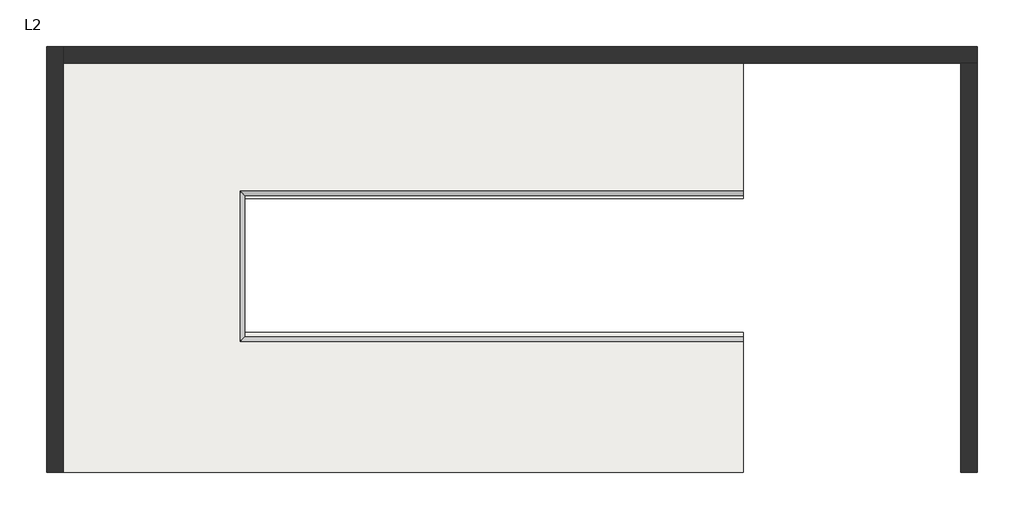
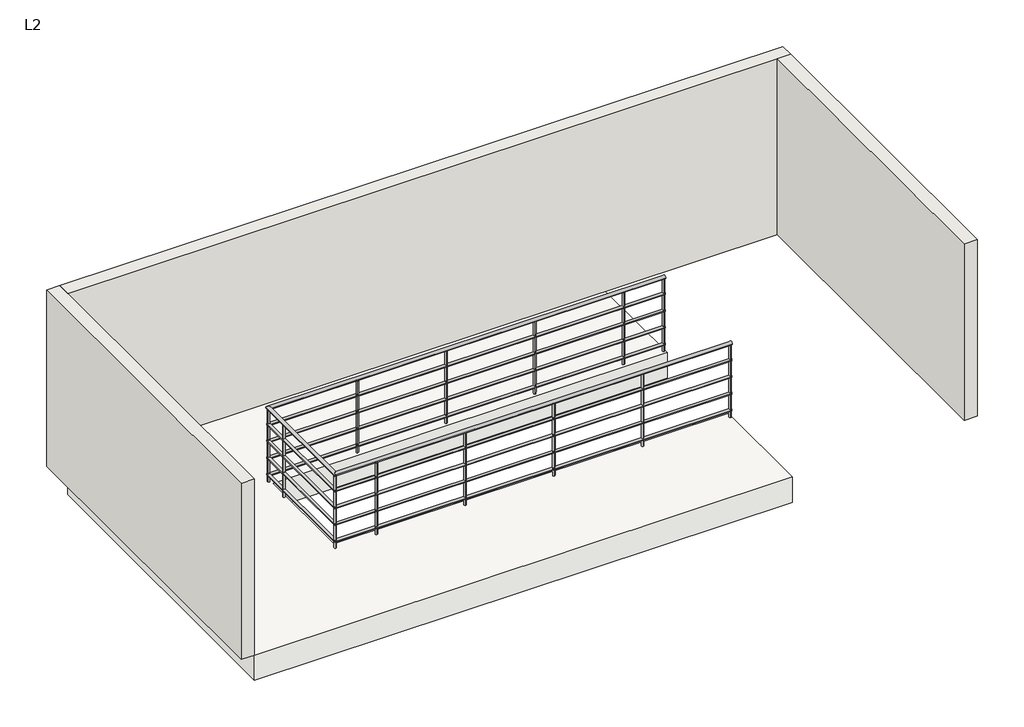
# One storey: 3 walls, 1 railing, 1 slab.
"""IFC4 building model written with IfcOpenShell, lengths in millimetres."""

from ifc_helpers import new_model, si_unit, point, frame, frame_2d, origin, place, context, project, spatial, polyline, circle_curve, ellipse_curve, trimmed, segment, composite_curve, outline, extrude, faceted_brep, element, save
from ifc_brep_helpers import plane_surface, cylinder_surface, advanced_brep

model = new_model("IFC4")

# Units and contexts
model_context = context("Model", 3, world=origin())
ifc_project = project(units=[si_unit("LENGTHUNIT", "METRE", prefix="MILLI")], contexts=[model_context])

# Site, building, storey
site = spatial("IfcSite", under=ifc_project)
building = spatial("IfcBuilding", under=site)
storey = spatial("IfcBuildingStorey", under=building, Name="L2", Elevation=2700.0)

# Railing
placement = place(None, origin())
element("IfcRailing", 1, ObjectType="900mm Pipe", at=placement, inside=storey, context=model_context, shape_type="SolidModel", body=[
    advanced_brep(
    [(-2164.8480531, 1633.4805305, 3580.0), (-2164.8480531, 1593.4805305, 3580.0), (-6608.8480531, 1633.4805305, 3580.0), (-6648.8480531, 1593.4805305, 3580.0), (-6608.8480531, 2893.4805305, 3580.0), (-6648.8480531, 2933.4805305, 3580.0), (-2164.8480531, 2893.4805305, 3580.0), (-2164.8480531, 2933.4805305, 3580.0)],
    [
        (0, 1, circle_curve(frame((-2164.8480531, 1613.4805305, 3580.0), z_axis=(1.0, 0.0, 0.0), x_axis=(0.0, -1.0, 0.0)), 20.0)),
        (1, 0, circle_curve(frame((-2164.8480531, 1613.4805305, 3580.0), z_axis=(1.0, 0.0, 0.0), x_axis=(0.0, -1.0, 0.0)), 20.0)),
        (0, 2),
        (2, 3, ellipse_curve(frame((-6628.8480531, 1613.4805305, 3580.0), z_axis=(0.7071067811865459, -0.7071067811865491, 0.0), x_axis=(0.7071067811865491, 0.7071067811865459, 0.0)), 28.2842712, 20.0)),
        (3, 1),
        (3, 2, ellipse_curve(frame((-6628.8480531, 1613.4805305, 3580.0), z_axis=(0.7071067811865459, -0.7071067811865491, 0.0), x_axis=(0.7071067811865491, 0.7071067811865459, 0.0)), 28.2842712, 20.0)),
        (2, 4),
        (4, 5, ellipse_curve(frame((-6628.8480531, 2913.4805305, 3580.0), z_axis=(-0.7071067811865492, -0.7071067811865458, 0.0), x_axis=(0.7071067811865457, -0.7071067811865493, 0.0)), 28.2842712, 20.0)),
        (5, 3),
        (5, 4, ellipse_curve(frame((-6628.8480531, 2913.4805305, 3580.0), z_axis=(-0.7071067811865492, -0.7071067811865458, 0.0), x_axis=(0.7071067811865457, -0.7071067811865493, 0.0)), 28.2842712, 20.0)),
        (6, 7, circle_curve(frame((-2164.8480531, 2913.4805305, 3580.0), z_axis=(1.0, 0.0, 0.0), x_axis=(0.0, 1.0, 0.0)), 20.0)),
        (7, 6, circle_curve(frame((-2164.8480531, 2913.4805305, 3580.0), z_axis=(1.0, 0.0, 0.0), x_axis=(0.0, 1.0, 0.0)), 20.0)),
        (4, 6),
        (7, 5),
    ],
    [
        plane_surface(frame((-2164.8480531, 1613.4805305, 3600.0), z_axis=(1.0, 0.0, 0.0), x_axis=(0.0, -1.0, 0.0))),
        cylinder_surface(frame((-2164.8480531, 1613.4805305, 3580.0), z_axis=(1.0, 0.0, 0.0), x_axis=(0.0, -1.0, 0.0)), 20.0),
        cylinder_surface(frame((-6628.8480531, 1613.4805305, 3580.0), z_axis=(0.0, -1.0, 0.0), x_axis=(-1.0, 0.0, 0.0)), 20.0),
        plane_surface(frame((-2164.8480531, 2913.4805305, 3600.0), z_axis=(1.0, 0.0, 0.0), x_axis=(0.0, 1.0, 0.0))),
        cylinder_surface(frame((-6628.8480531, 2913.4805305, 3580.0), z_axis=(-1.0, 0.0, 0.0), x_axis=(0.0, 1.0, 0.0)), 20.0),
    ],
    [
        (0, [[1, 2]]),
        (1, [[-1, 3, 4, 5]]),
        (1, [[-2, -5, 6, -3]]),
        (2, [[-4, 7, 8, 9]]),
        (2, [[-6, -9, 10, -7]]),
        (3, [[11, 12]]),
        (4, [[-8, 13, -12, 14]]),
        (4, [[-10, -14, -11, -13]]),
    ],
),
    advanced_brep(
    [(-2164.8480531, 1598.4805305, 3385.0), (-2164.8480531, 1628.4805305, 3385.0), (-6643.8480531, 1598.4805305, 3385.0), (-6613.8480531, 1628.4805305, 3385.0), (-6643.8480531, 2928.4805305, 3385.0), (-6613.8480531, 2898.4805305, 3385.0), (-2164.8480531, 2928.4805305, 3385.0), (-2164.8480531, 2898.4805305, 3385.0)],
    [
        (0, 1, circle_curve(frame((-2164.8480531, 1613.4805305, 3385.0), z_axis=(1.0, 0.0, 0.0), x_axis=(0.0, 1.0, 0.0)), 15.0)),
        (1, 0, circle_curve(frame((-2164.8480531, 1613.4805305, 3385.0), z_axis=(1.0, 0.0, 0.0), x_axis=(0.0, 1.0, 0.0)), 15.0)),
        (0, 2),
        (2, 3, ellipse_curve(frame((-6628.8480531, 1613.4805305, 3385.0), z_axis=(0.7071067811865459, -0.7071067811865491, 0.0), x_axis=(0.7071067811865491, 0.7071067811865459, 0.0)), 21.2132034, 15.0)),
        (3, 1),
        (3, 2, ellipse_curve(frame((-6628.8480531, 1613.4805305, 3385.0), z_axis=(0.7071067811865459, -0.7071067811865491, 0.0), x_axis=(0.7071067811865491, 0.7071067811865459, 0.0)), 21.2132034, 15.0)),
        (2, 4),
        (4, 5, ellipse_curve(frame((-6628.8480531, 2913.4805305, 3385.0), z_axis=(-0.7071067811865492, -0.7071067811865458, 0.0), x_axis=(0.7071067811865457, -0.7071067811865493, 0.0)), 21.2132034, 15.0)),
        (5, 3),
        (5, 4, ellipse_curve(frame((-6628.8480531, 2913.4805305, 3385.0), z_axis=(-0.7071067811865492, -0.7071067811865458, 0.0), x_axis=(0.7071067811865457, -0.7071067811865493, 0.0)), 21.2132034, 15.0)),
        (6, 7, circle_curve(frame((-2164.8480531, 2913.4805305, 3385.0), z_axis=(1.0, 0.0, 0.0), x_axis=(0.0, -1.0, 0.0)), 15.0)),
        (7, 6, circle_curve(frame((-2164.8480531, 2913.4805305, 3385.0), z_axis=(1.0, 0.0, 0.0), x_axis=(0.0, -1.0, 0.0)), 15.0)),
        (4, 6),
        (7, 5),
    ],
    [
        plane_surface(frame((-2164.8480531, 1613.4805305, 3400.0), z_axis=(1.0, 0.0, 0.0), x_axis=(0.0, -1.0, 0.0))),
        cylinder_surface(frame((-2164.8480531, 1613.4805305, 3385.0), z_axis=(1.0, 0.0, 0.0), x_axis=(0.0, 1.0, 0.0)), 15.0),
        cylinder_surface(frame((-6628.8480531, 1613.4805305, 3385.0), z_axis=(0.0, -1.0, 0.0), x_axis=(1.0, 0.0, 0.0)), 15.0),
        plane_surface(frame((-2164.8480531, 2913.4805305, 3400.0), z_axis=(1.0, 0.0, 0.0), x_axis=(0.0, 1.0, 0.0))),
        cylinder_surface(frame((-6628.8480531, 2913.4805305, 3385.0), z_axis=(-1.0, 0.0, 0.0), x_axis=(0.0, -1.0, 0.0)), 15.0),
    ],
    [
        (0, [[1, 2]]),
        (1, [[-1, 3, 4, 5]]),
        (1, [[-2, -5, 6, -3]]),
        (2, [[-4, 7, 8, 9]]),
        (2, [[-6, -9, 10, -7]]),
        (3, [[11, 12]]),
        (4, [[-8, 13, -12, 14]]),
        (4, [[-10, -14, -11, -13]]),
    ],
),
    advanced_brep(
    [(-2164.8480531, 1598.4805305, 3185.0), (-2164.8480531, 1628.4805305, 3185.0), (-6643.8480531, 1598.4805305, 3185.0), (-6613.8480531, 1628.4805305, 3185.0), (-6643.8480531, 2928.4805305, 3185.0), (-6613.8480531, 2898.4805305, 3185.0), (-2164.8480531, 2928.4805305, 3185.0), (-2164.8480531, 2898.4805305, 3185.0)],
    [
        (0, 1, circle_curve(frame((-2164.8480531, 1613.4805305, 3185.0), z_axis=(1.0, 0.0, 0.0), x_axis=(0.0, 1.0, 0.0)), 15.0)),
        (1, 0, circle_curve(frame((-2164.8480531, 1613.4805305, 3185.0), z_axis=(1.0, 0.0, 0.0), x_axis=(0.0, 1.0, 0.0)), 15.0)),
        (0, 2),
        (2, 3, ellipse_curve(frame((-6628.8480531, 1613.4805305, 3185.0), z_axis=(0.7071067811865459, -0.7071067811865491, 0.0), x_axis=(0.7071067811865491, 0.7071067811865459, 0.0)), 21.2132034, 15.0)),
        (3, 1),
        (3, 2, ellipse_curve(frame((-6628.8480531, 1613.4805305, 3185.0), z_axis=(0.7071067811865459, -0.7071067811865491, 0.0), x_axis=(0.7071067811865491, 0.7071067811865459, 0.0)), 21.2132034, 15.0)),
        (2, 4),
        (4, 5, ellipse_curve(frame((-6628.8480531, 2913.4805305, 3185.0), z_axis=(-0.7071067811865492, -0.7071067811865458, 0.0), x_axis=(0.7071067811865457, -0.7071067811865493, 0.0)), 21.2132034, 15.0)),
        (5, 3),
        (5, 4, ellipse_curve(frame((-6628.8480531, 2913.4805305, 3185.0), z_axis=(-0.7071067811865492, -0.7071067811865458, 0.0), x_axis=(0.7071067811865457, -0.7071067811865493, 0.0)), 21.2132034, 15.0)),
        (6, 7, circle_curve(frame((-2164.8480531, 2913.4805305, 3185.0), z_axis=(1.0, 0.0, 0.0), x_axis=(0.0, -1.0, 0.0)), 15.0)),
        (7, 6, circle_curve(frame((-2164.8480531, 2913.4805305, 3185.0), z_axis=(1.0, 0.0, 0.0), x_axis=(0.0, -1.0, 0.0)), 15.0)),
        (4, 6),
        (7, 5),
    ],
    [
        plane_surface(frame((-2164.8480531, 1613.4805305, 3200.0), z_axis=(1.0, 0.0, 0.0), x_axis=(0.0, -1.0, 0.0))),
        cylinder_surface(frame((-2164.8480531, 1613.4805305, 3185.0), z_axis=(1.0, 0.0, 0.0), x_axis=(0.0, 1.0, 0.0)), 15.0),
        cylinder_surface(frame((-6628.8480531, 1613.4805305, 3185.0), z_axis=(0.0, -1.0, 0.0), x_axis=(1.0, 0.0, 0.0)), 15.0),
        plane_surface(frame((-2164.8480531, 2913.4805305, 3200.0), z_axis=(1.0, 0.0, 0.0), x_axis=(0.0, 1.0, 0.0))),
        cylinder_surface(frame((-6628.8480531, 2913.4805305, 3185.0), z_axis=(-1.0, 0.0, 0.0), x_axis=(0.0, -1.0, 0.0)), 15.0),
    ],
    [
        (0, [[1, 2]]),
        (1, [[-1, 3, 4, 5]]),
        (1, [[-2, -5, 6, -3]]),
        (2, [[-4, 7, 8, 9]]),
        (2, [[-6, -9, 10, -7]]),
        (3, [[11, 12]]),
        (4, [[-8, 13, -12, 14]]),
        (4, [[-10, -14, -11, -13]]),
    ],
),
    advanced_brep(
    [(-2164.8480531, 1598.4805305, 2985.0), (-2164.8480531, 1628.4805305, 2985.0), (-6643.8480531, 1598.4805305, 2985.0), (-6613.8480531, 1628.4805305, 2985.0), (-6643.8480531, 2928.4805305, 2985.0), (-6613.8480531, 2898.4805305, 2985.0), (-2164.8480531, 2928.4805305, 2985.0), (-2164.8480531, 2898.4805305, 2985.0)],
    [
        (0, 1, circle_curve(frame((-2164.8480531, 1613.4805305, 2985.0), z_axis=(1.0, 0.0, 0.0), x_axis=(0.0, 1.0, 0.0)), 15.0)),
        (1, 0, circle_curve(frame((-2164.8480531, 1613.4805305, 2985.0), z_axis=(1.0, 0.0, 0.0), x_axis=(0.0, 1.0, 0.0)), 15.0)),
        (0, 2),
        (2, 3, ellipse_curve(frame((-6628.8480531, 1613.4805305, 2985.0), z_axis=(0.7071067811865459, -0.7071067811865491, 0.0), x_axis=(0.7071067811865491, 0.7071067811865459, 0.0)), 21.2132034, 15.0)),
        (3, 1),
        (3, 2, ellipse_curve(frame((-6628.8480531, 1613.4805305, 2985.0), z_axis=(0.7071067811865459, -0.7071067811865491, 0.0), x_axis=(0.7071067811865491, 0.7071067811865459, 0.0)), 21.2132034, 15.0)),
        (2, 4),
        (4, 5, ellipse_curve(frame((-6628.8480531, 2913.4805305, 2985.0), z_axis=(-0.7071067811865492, -0.7071067811865458, 0.0), x_axis=(0.7071067811865457, -0.7071067811865493, 0.0)), 21.2132034, 15.0)),
        (5, 3),
        (5, 4, ellipse_curve(frame((-6628.8480531, 2913.4805305, 2985.0), z_axis=(-0.7071067811865492, -0.7071067811865458, 0.0), x_axis=(0.7071067811865457, -0.7071067811865493, 0.0)), 21.2132034, 15.0)),
        (6, 7, circle_curve(frame((-2164.8480531, 2913.4805305, 2985.0), z_axis=(1.0, 0.0, 0.0), x_axis=(0.0, -1.0, 0.0)), 15.0)),
        (7, 6, circle_curve(frame((-2164.8480531, 2913.4805305, 2985.0), z_axis=(1.0, 0.0, 0.0), x_axis=(0.0, -1.0, 0.0)), 15.0)),
        (4, 6),
        (7, 5),
    ],
    [
        plane_surface(frame((-2164.8480531, 1613.4805305, 3000.0), z_axis=(1.0, 0.0, 0.0), x_axis=(0.0, -1.0, 0.0))),
        cylinder_surface(frame((-2164.8480531, 1613.4805305, 2985.0), z_axis=(1.0, 0.0, 0.0), x_axis=(0.0, 1.0, 0.0)), 15.0),
        cylinder_surface(frame((-6628.8480531, 1613.4805305, 2985.0), z_axis=(0.0, -1.0, 0.0), x_axis=(1.0, 0.0, 0.0)), 15.0),
        plane_surface(frame((-2164.8480531, 2913.4805305, 3000.0), z_axis=(1.0, 0.0, 0.0), x_axis=(0.0, 1.0, 0.0))),
        cylinder_surface(frame((-6628.8480531, 2913.4805305, 2985.0), z_axis=(-1.0, 0.0, 0.0), x_axis=(0.0, -1.0, 0.0)), 15.0),
    ],
    [
        (0, [[1, 2]]),
        (1, [[-1, 3, 4, 5]]),
        (1, [[-2, -5, 6, -3]]),
        (2, [[-4, 7, 8, 9]]),
        (2, [[-6, -9, 10, -7]]),
        (3, [[11, 12]]),
        (4, [[-8, 13, -12, 14]]),
        (4, [[-10, -14, -11, -13]]),
    ],
),
    advanced_brep(
    [(-2164.8480531, 1598.4805305, 2785.0), (-2164.8480531, 1628.4805305, 2785.0), (-6643.8480531, 1598.4805305, 2785.0), (-6613.8480531, 1628.4805305, 2785.0), (-6643.8480531, 2928.4805305, 2785.0), (-6613.8480531, 2898.4805305, 2785.0), (-2164.8480531, 2928.4805305, 2785.0), (-2164.8480531, 2898.4805305, 2785.0)],
    [
        (0, 1, circle_curve(frame((-2164.8480531, 1613.4805305, 2785.0), z_axis=(1.0, 0.0, 0.0), x_axis=(0.0, 1.0, 0.0)), 15.0)),
        (1, 0, circle_curve(frame((-2164.8480531, 1613.4805305, 2785.0), z_axis=(1.0, 0.0, 0.0), x_axis=(0.0, 1.0, 0.0)), 15.0)),
        (0, 2),
        (2, 3, ellipse_curve(frame((-6628.8480531, 1613.4805305, 2785.0), z_axis=(0.7071067811865459, -0.7071067811865491, 0.0), x_axis=(0.7071067811865491, 0.7071067811865459, 0.0)), 21.2132034, 15.0)),
        (3, 1),
        (3, 2, ellipse_curve(frame((-6628.8480531, 1613.4805305, 2785.0), z_axis=(0.7071067811865459, -0.7071067811865491, 0.0), x_axis=(0.7071067811865491, 0.7071067811865459, 0.0)), 21.2132034, 15.0)),
        (2, 4),
        (4, 5, ellipse_curve(frame((-6628.8480531, 2913.4805305, 2785.0), z_axis=(-0.7071067811865492, -0.7071067811865458, 0.0), x_axis=(0.7071067811865457, -0.7071067811865493, 0.0)), 21.2132034, 15.0)),
        (5, 3),
        (5, 4, ellipse_curve(frame((-6628.8480531, 2913.4805305, 2785.0), z_axis=(-0.7071067811865492, -0.7071067811865458, 0.0), x_axis=(0.7071067811865457, -0.7071067811865493, 0.0)), 21.2132034, 15.0)),
        (6, 7, circle_curve(frame((-2164.8480531, 2913.4805305, 2785.0), z_axis=(1.0, 0.0, 0.0), x_axis=(0.0, -1.0, 0.0)), 15.0)),
        (7, 6, circle_curve(frame((-2164.8480531, 2913.4805305, 2785.0), z_axis=(1.0, 0.0, 0.0), x_axis=(0.0, -1.0, 0.0)), 15.0)),
        (4, 6),
        (7, 5),
    ],
    [
        plane_surface(frame((-2164.8480531, 1613.4805305, 2800.0), z_axis=(1.0, 0.0, 0.0), x_axis=(0.0, -1.0, 0.0))),
        cylinder_surface(frame((-2164.8480531, 1613.4805305, 2785.0), z_axis=(1.0, 0.0, 0.0), x_axis=(0.0, 1.0, 0.0)), 15.0),
        cylinder_surface(frame((-6628.8480531, 1613.4805305, 2785.0), z_axis=(0.0, -1.0, 0.0), x_axis=(1.0, 0.0, 0.0)), 15.0),
        plane_surface(frame((-2164.8480531, 2913.4805305, 2800.0), z_axis=(1.0, 0.0, 0.0), x_axis=(0.0, 1.0, 0.0))),
        cylinder_surface(frame((-6628.8480531, 2913.4805305, 2785.0), z_axis=(-1.0, 0.0, 0.0), x_axis=(0.0, -1.0, 0.0)), 15.0),
    ],
    [
        (0, [[1, 2]]),
        (1, [[-1, 3, 4, 5]]),
        (1, [[-2, -5, 6, -3]]),
        (2, [[-4, 7, 8, 9]]),
        (2, [[-6, -9, 10, -7]]),
        (3, [[11, 12]]),
        (4, [[-8, 13, -12, 14]]),
        (4, [[-10, -14, -11, -13]]),
    ],
),
    extrude(outline(composite_curve([segment(trimmed(circle_curve(frame_2d((-2628.8480531, 2913.4805305)), 12.5), [point((-2628.8480531, 2925.9805305))], [point((-2628.8480531, 2900.9805305))], False, "CARTESIAN"), True, "CONTINUOUS"), segment(trimmed(circle_curve(frame_2d((-2628.8480531, 2913.4805305)), 12.5), [point((-2628.8480531, 2900.9805305))], [point((-2628.8480531, 2925.9805305))], False, "CARTESIAN"), True, "CONTINUOUS")], self_intersect=False)), frame((0.0, 0.0, 2700.0), z_axis=(0.0, 0.0, 1.0), x_axis=(1.0, 0.0, 0.0)), (0.0, 0.0, 1.0), 860.0),
    extrude(outline(composite_curve([segment(trimmed(circle_curve(frame_2d((-3628.8480531, 2913.4805305)), 12.5), [point((-3628.8480531, 2925.9805305))], [point((-3628.8480531, 2900.9805305))], False, "CARTESIAN"), True, "CONTINUOUS"), segment(trimmed(circle_curve(frame_2d((-3628.8480531, 2913.4805305)), 12.5), [point((-3628.8480531, 2900.9805305))], [point((-3628.8480531, 2925.9805305))], False, "CARTESIAN"), True, "CONTINUOUS")], self_intersect=False)), frame((0.0, 0.0, 2700.0), z_axis=(0.0, 0.0, 1.0), x_axis=(1.0, 0.0, 0.0)), (0.0, 0.0, 1.0), 860.0),
    extrude(outline(composite_curve([segment(trimmed(circle_curve(frame_2d((-4628.8480531, 2913.4805305)), 12.5), [point((-4628.8480531, 2925.9805305))], [point((-4628.8480531, 2900.9805305))], False, "CARTESIAN"), True, "CONTINUOUS"), segment(trimmed(circle_curve(frame_2d((-4628.8480531, 2913.4805305)), 12.5), [point((-4628.8480531, 2900.9805305))], [point((-4628.8480531, 2925.9805305))], False, "CARTESIAN"), True, "CONTINUOUS")], self_intersect=False)), frame((0.0, 0.0, 2700.0), z_axis=(0.0, 0.0, 1.0), x_axis=(1.0, 0.0, 0.0)), (0.0, 0.0, 1.0), 860.0),
    extrude(outline(composite_curve([segment(trimmed(circle_curve(frame_2d((-5628.8480531, 2913.4805305)), 12.5), [point((-5628.8480531, 2925.9805305))], [point((-5628.8480531, 2900.9805305))], False, "CARTESIAN"), True, "CONTINUOUS"), segment(trimmed(circle_curve(frame_2d((-5628.8480531, 2913.4805305)), 12.5), [point((-5628.8480531, 2900.9805305))], [point((-5628.8480531, 2925.9805305))], False, "CARTESIAN"), True, "CONTINUOUS")], self_intersect=False)), frame((0.0, 0.0, 2700.0), z_axis=(0.0, 0.0, 1.0), x_axis=(1.0, 0.0, 0.0)), (0.0, 0.0, 1.0), 860.0),
    extrude(outline(composite_curve([segment(trimmed(circle_curve(frame_2d((-6628.8480531, 2613.4805305)), 12.5), [point((-6641.3480531, 2613.4805305))], [point((-6616.3480531, 2613.4805305))], False, "CARTESIAN"), True, "CONTINUOUS"), segment(trimmed(circle_curve(frame_2d((-6628.8480531, 2613.4805305)), 12.5), [point((-6616.3480531, 2613.4805305))], [point((-6641.3480531, 2613.4805305))], False, "CARTESIAN"), True, "CONTINUOUS")], self_intersect=False)), frame((0.0, 0.0, 2700.0), z_axis=(0.0, 0.0, 1.0), x_axis=(1.0, 0.0, 0.0)), (0.0, 0.0, 1.0), 860.0),
    extrude(outline(composite_curve([segment(trimmed(circle_curve(frame_2d((-6164.8480531, 1613.4805305)), 12.5), [point((-6164.8480531, 1600.9805305))], [point((-6164.8480531, 1625.9805305))], False, "CARTESIAN"), True, "CONTINUOUS"), segment(trimmed(circle_curve(frame_2d((-6164.8480531, 1613.4805305)), 12.5), [point((-6164.8480531, 1625.9805305))], [point((-6164.8480531, 1600.9805305))], False, "CARTESIAN"), True, "CONTINUOUS")], self_intersect=False)), frame((0.0, 0.0, 2700.0), z_axis=(0.0, 0.0, 1.0), x_axis=(1.0, 0.0, 0.0)), (0.0, 0.0, 1.0), 860.0),
    extrude(outline(composite_curve([segment(trimmed(circle_curve(frame_2d((-5164.8480531, 1613.4805305)), 12.5), [point((-5164.8480531, 1600.9805305))], [point((-5164.8480531, 1625.9805305))], False, "CARTESIAN"), True, "CONTINUOUS"), segment(trimmed(circle_curve(frame_2d((-5164.8480531, 1613.4805305)), 12.5), [point((-5164.8480531, 1625.9805305))], [point((-5164.8480531, 1600.9805305))], False, "CARTESIAN"), True, "CONTINUOUS")], self_intersect=False)), frame((0.0, 0.0, 2700.0), z_axis=(0.0, 0.0, 1.0), x_axis=(1.0, 0.0, 0.0)), (0.0, 0.0, 1.0), 860.0),
    extrude(outline(composite_curve([segment(trimmed(circle_curve(frame_2d((-4164.8480531, 1613.4805305)), 12.5), [point((-4164.8480531, 1600.9805305))], [point((-4164.8480531, 1625.9805305))], False, "CARTESIAN"), True, "CONTINUOUS"), segment(trimmed(circle_curve(frame_2d((-4164.8480531, 1613.4805305)), 12.5), [point((-4164.8480531, 1625.9805305))], [point((-4164.8480531, 1600.9805305))], False, "CARTESIAN"), True, "CONTINUOUS")], self_intersect=False)), frame((0.0, 0.0, 2700.0), z_axis=(0.0, 0.0, 1.0), x_axis=(1.0, 0.0, 0.0)), (0.0, 0.0, 1.0), 860.0),
    extrude(outline(composite_curve([segment(trimmed(circle_curve(frame_2d((-3164.8480531, 1613.4805305)), 12.5), [point((-3164.8480531, 1600.9805305))], [point((-3164.8480531, 1625.9805305))], False, "CARTESIAN"), True, "CONTINUOUS"), segment(trimmed(circle_curve(frame_2d((-3164.8480531, 1613.4805305)), 12.5), [point((-3164.8480531, 1625.9805305))], [point((-3164.8480531, 1600.9805305))], False, "CARTESIAN"), True, "CONTINUOUS")], self_intersect=False)), frame((0.0, 0.0, 2700.0), z_axis=(0.0, 0.0, 1.0), x_axis=(1.0, 0.0, 0.0)), (0.0, 0.0, 1.0), 860.0),
    extrude(outline(composite_curve([segment(trimmed(circle_curve(frame_2d((-6628.8480531, 2913.4805305)), 12.5), [point((-6641.3480531, 2913.4805305))], [point((-6616.3480531, 2913.4805305))], False, "CARTESIAN"), True, "CONTINUOUS"), segment(trimmed(circle_curve(frame_2d((-6628.8480531, 2913.4805305)), 12.5), [point((-6616.3480531, 2913.4805305))], [point((-6641.3480531, 2913.4805305))], False, "CARTESIAN"), True, "CONTINUOUS")], self_intersect=False)), frame((0.0, 0.0, 2700.0), z_axis=(0.0, 0.0, 1.0), x_axis=(1.0, 0.0, 0.0)), (0.0, 0.0, 1.0), 860.0),
    extrude(outline(composite_curve([segment(trimmed(circle_curve(frame_2d((-6628.8480531, 1613.4805305)), 12.5), [point((-6628.8480531, 1600.9805305))], [point((-6628.8480531, 1625.9805305))], False, "CARTESIAN"), True, "CONTINUOUS"), segment(trimmed(circle_curve(frame_2d((-6628.8480531, 1613.4805305)), 12.5), [point((-6628.8480531, 1625.9805305))], [point((-6628.8480531, 1600.9805305))], False, "CARTESIAN"), True, "CONTINUOUS")], self_intersect=False)), frame((0.0, 0.0, 2700.0), z_axis=(0.0, 0.0, 1.0), x_axis=(1.0, 0.0, 0.0)), (0.0, 0.0, 1.0), 860.0),
    extrude(outline(composite_curve([segment(trimmed(circle_curve(frame_2d((-2177.3480531, 2913.4805305)), 12.5), [point((-2177.3480531, 2925.9805305))], [point((-2177.3480531, 2900.9805305))], False, "CARTESIAN"), True, "CONTINUOUS"), segment(trimmed(circle_curve(frame_2d((-2177.3480531, 2913.4805305)), 12.5), [point((-2177.3480531, 2900.9805305))], [point((-2177.3480531, 2925.9805305))], False, "CARTESIAN"), True, "CONTINUOUS")], self_intersect=False)), frame((0.0, 0.0, 2700.0), z_axis=(0.0, 0.0, 1.0), x_axis=(1.0, 0.0, 0.0)), (0.0, 0.0, 1.0), 860.0),
    extrude(outline(composite_curve([segment(trimmed(circle_curve(frame_2d((-2177.3480531, 1613.4805305)), 12.5), [point((-2177.3480531, 1600.9805305))], [point((-2177.3480531, 1625.9805305))], False, "CARTESIAN"), True, "CONTINUOUS"), segment(trimmed(circle_curve(frame_2d((-2177.3480531, 1613.4805305)), 12.5), [point((-2177.3480531, 1625.9805305))], [point((-2177.3480531, 1600.9805305))], False, "CARTESIAN"), True, "CONTINUOUS")], self_intersect=False)), frame((0.0, 0.0, 2700.0), z_axis=(0.0, 0.0, 1.0), x_axis=(1.0, 0.0, 0.0)), (0.0, 0.0, 1.0), 860.0),
])

# Slab
element("IfcSlab", 2, ObjectType="Generic 300mm", at=placement, inside=storey, context=model_context, shape_type="SweptSolid", body=[
    extrude(outline(polyline([(-8225.0, 4075.0), (-5925.0, 4075.0), (-2161.0, 4075.0), (-2161.0, 2869.6), (-6608.8480531, 2869.6), (-6608.8480531, 1675.0), (-2161.0, 1675.0), (-2161.0, 425.0), (-8225.0, 425.0), (-8225.0, 4075.0)])), frame((0.0, 0.0, 2400.0), z_axis=(0.0, 0.0, 1.0), x_axis=(1.0, 0.0, 0.0)), (0.0, 0.0, 1.0), 300.0),
])

# Walls
element("IfcWall", 3, ObjectType="Generic - 150mm", at=placement, inside=storey, context=model_context, shape_type="Brep", body=[
    faceted_brep([(-8225.0, 425.0, 2700.0), (-8225.0, 4075.0, 2700.0), (-8225.0, 4225.0, 2700.0), (-8225.0, 4225.0, 4800.0), (-8225.0, 4075.0, 4800.0), (-8225.0, 425.0, 4800.0), (-8375.0, 425.0, 2700.0), (-8375.0, 425.0, 4800.0), (-8375.0, 4225.0, 4800.0), (-8375.0, 4225.0, 2700.0)], [[[0, 1, 2, 3, 4, 5]], [[6, 7, 8, 9]], [[2, 1, 0, 6, 9]], [[5, 4, 3, 8, 7]], [[0, 5, 7, 6]], [[3, 2, 9, 8]]]),
])
element("IfcWall", 4, ObjectType="Generic - 150mm", at=placement, inside=storey, context=model_context, shape_type="Brep", body=[
    faceted_brep([(-8225.0, 4075.0, 2700.0), (-225.0, 4075.0, 2700.0), (-75.0, 4075.0, 2700.0), (-75.0, 4075.0, 4800.0), (-225.0, 4075.0, 4800.0), (-8225.0, 4075.0, 4800.0), (-8225.0, 4225.0, 2700.0), (-8225.0, 4225.0, 4800.0), (-75.0, 4225.0, 4800.0), (-75.0, 4225.0, 2700.0)], [[[0, 1, 2, 3, 4, 5]], [[6, 7, 8, 9]], [[2, 1, 0, 6, 9]], [[5, 4, 3, 8, 7]], [[0, 5, 7, 6]], [[3, 2, 9, 8]]]),
])
element("IfcWall", 5, ObjectType="Generic - 150mm", at=placement, inside=storey, context=model_context, shape_type="SweptSolid", body=[
    extrude(outline(polyline([(-225.0, 425.0), (-225.0, 4075.0), (-75.0, 4075.0), (-75.0, 425.0), (-225.0, 425.0)])), frame((0.0, 0.0, 2700.0), z_axis=(0.0, 0.0, 1.0), x_axis=(1.0, 0.0, 0.0)), (0.0, 0.0, 1.0), 2100.0),
])

save(model, "model.ifc")

# Revit data of these elements
# Project information
#   Название организации = "Organization Name"
#   Описание организации = "Organization Description"
#   Наименование здания = "Building Name"
#   Дата утверждения проекта = "Issue Date"
#   Статус проекта = "Project Status"
#   Заказчик = "Client Name"
#   Адрес проекта = "Enter address here\nAddress Line 2"
#   Наименование проекта = "Project Name"
#   Номер проекта = "Project Number"
# Type "900mm Pipe"
#   built-in parameter 1008612 = 0.019685 (stored number, unit not read)
#   built-in parameter 1008611 = 0.0984252 (stored number, unit not read)
#   built-in parameter 1008609 = 3.28084 (stored number, unit not read)
#   built-in parameter 1008604 = 0.19685 (stored number, unit not read)
#   built-in parameter 1008603 = 0.164042 (stored number, unit not read)
#   Railing Height = 900 mm
#   built-in parameter 1008630 = 2
#   built-in parameter 1008610 = 1
#   built-in parameter 1008605 = 1
#   built-in parameter 1008618 = M_Baluster - Round : 25mm
# Type "Generic 300mm"
#   Description = "Generic Floor (Material By Category), 300mm thick"
#   Function = 0
#   Layers, outside or top first: 300 mm no material (function 1)
# Type "Generic - 150mm"
#   Description = "Generic Wall (Material By Category), 150mm thick"
#   Type Mark = "G04"
#   Layers, outside or top first: 150 mm no material (function 1)
# Element 1 (IfcRailing, "900mm Pipe")
#   Phase Created = New Construction
# Element 2 (IfcSlab, "Generic 300mm")
#   Height Offset From Level = 0 mm
#   Phase Created = New Construction
#   Materials on its faces: "Default Floor"
# Elements 3, 4, 5 (IfcWall, "Generic - 150mm")
#   Top Offset = 0 mm
#   Base Offset = 0 mm
#   Unconnected Height = 2100 mm
#   wall height = 2100 mm
#   Phase Created = New Construction
#   Base Constraint = L2
#   Materials on its faces: "Default Wall"
# Materials
#   "Default Floor": class "Miscellaneous", colour RGB 128 128 128, transparency 0, Cost = 0
#   "Default Wall": class "Miscellaneous", colour RGB 192 192 192, transparency 0, Cost = 0
